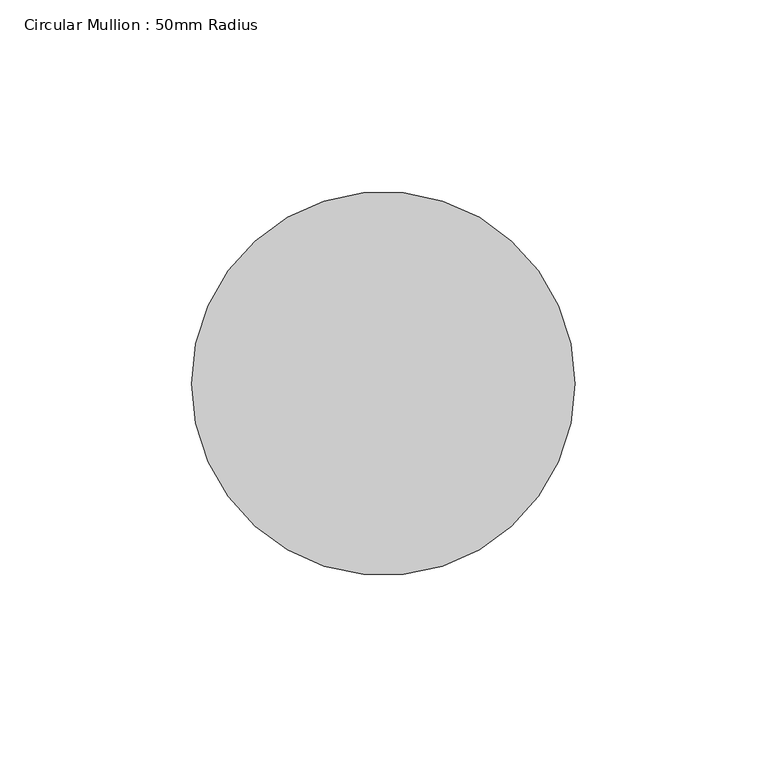
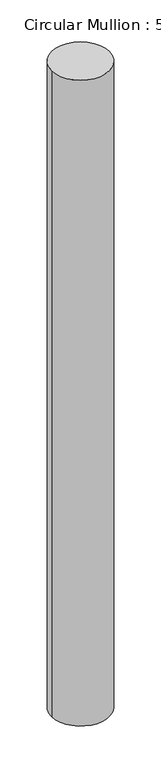
"""IFC4 building model written with IfcOpenShell, lengths in millimetres: member geometry, Circular Mullion : 50mm Radius."""

from ifc_helpers import new_model, si_unit, point, frame, origin, origin_2d, place, context, project, spatial, circle_curve, trimmed, segment, composite_curve, outline, extrude, source, transform, mapped, element, save


def circular_mullion_50mm_radius_d75af731(model_context):
    return source(origin(), model_context, "Body", "SweptSolid", [
        extrude(outline(composite_curve([segment(trimmed(circle_curve(origin_2d(), 50.0), [point((50.0, 0.0))], [point((-50.0, 0.0))], False, "CARTESIAN"), True, "CONTINUOUS"), segment(trimmed(circle_curve(origin_2d(), 50.0), [point((-50.0, 0.0))], [point((50.0, 0.0))], False, "CARTESIAN"), True, "CONTINUOUS")], self_intersect=False)), frame((0.0, 0.0, -1181.3150436), z_axis=(0.0, 0.0, 1.0), x_axis=(1.0, 0.0, 0.0)), (0.0, 0.0, 1.0), 1181.3150436),
    ])


if __name__ == "__main__":
    model = new_model("IFC4")
    model_context = context("Model", 3, world=origin())
    ifc_project = project(units=[si_unit("LENGTHUNIT", "METRE", prefix="MILLI")], contexts=[model_context])
    site = spatial("IfcSite", under=ifc_project)
    building = spatial("IfcBuilding", under=site)
    placement = place(None, origin())
    circular_mullion_50mm_radius_shape = circular_mullion_50mm_radius_d75af731(model_context)
    element("IfcMember", 1, ObjectType="Circular Mullion : 50mm Radius", at=placement, inside=building, context=model_context, shape_type="MappedRepresentation", body=[
        mapped(circular_mullion_50mm_radius_shape, transform((0.0, 0.0, 0.0), x_axis=(1.0, 0.0, 0.0), y_axis=(0.0, 1.0, 0.0), z_axis=(0.0, 0.0, 1.0))),
    ])
    save(model, "model.ifc")

# Revit data of these elements
# Type "Circular Mullion : 50mm Radius"
#   built-in parameter 1007350 = 0.164042 (stored number, unit not read)
# Element 1 (IfcMember, "Circular Mullion : 50mm Radius")
#   Materials on its faces: "Aluminium"
# Materials
#   "Aluminium": class "Metal", colour RGB 247 247 247, transparency 0, Description = "Aluminium 6061", Cost = 0
